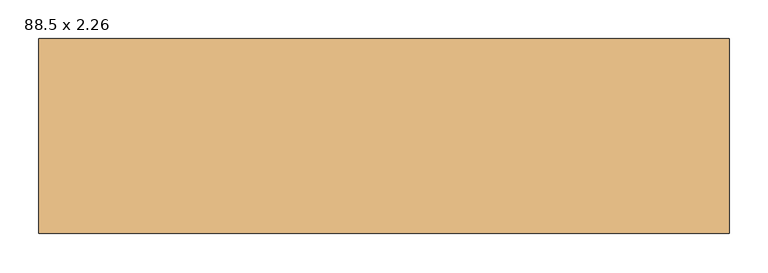
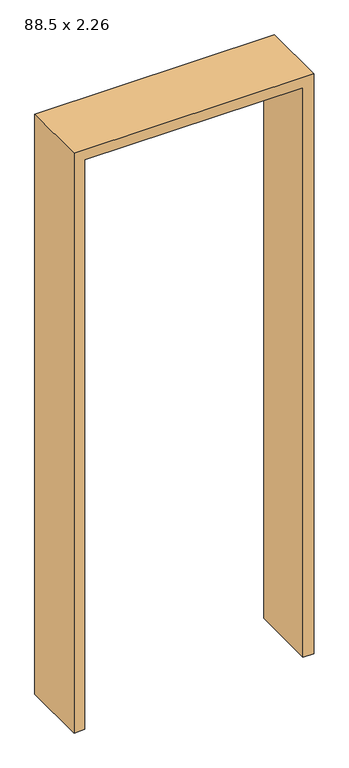
"""IFC4 building model written with IfcOpenShell, lengths in millimetres: door geometry, Durchfahrt - Blockzarge : 88.5 x 2.26."""

import ifcopenshell
import ifcopenshell.guid

model = None  # the IFC model being written
_history = None  # IfcOwnerHistory: only IFC2X3 demands one
_inside = {}  # id of a spatial element -> (the spatial element, [elements in it])
_under = {}  # id of a project, library or spatial element -> (it, [spatial elements below it])
_declared = {}  # id of a project -> (the project, [libraries it declares])
_typed = {}  # id of a type object -> (the type object, [elements of that type])
_made_of = {}  # id of a material, layer set ... -> (it, [elements and type objects made of it])


def new_model(schema):
    """Start an empty IFC model of exactly this schema.

    Asked for "IFC4X3", IfcOpenShell would pick the latest addendum, in which some entities
    have other attributes; the version numbers below select the first issue.
    IFC2X3 requires an IfcOwnerHistory on every rooted entity: one is made here for all.
    """
    global model, _history
    if schema == "IFC4X3":
        model = ifcopenshell.file(schema_version=(4, 3, 0, 0))
    else:
        model = ifcopenshell.file(schema=schema)
    _inside.clear()
    _under.clear()
    _declared.clear()
    _typed.clear()
    _made_of.clear()
    _history = None
    if model.schema == "IFC2X3":
        org = make("IfcOrganization", Name="unknown")
        user = make(
            "IfcPersonAndOrganization",
            ThePerson=make("IfcPerson", FamilyName="unknown"),
            TheOrganization=org,
        )
        app = make(
            "IfcApplication",
            ApplicationDeveloper=org,
            Version="unknown",
            ApplicationFullName="unknown",
            ApplicationIdentifier="unknown",
        )
        _history = make(
            "IfcOwnerHistory",
            OwningUser=user,
            OwningApplication=app,
            ChangeAction="ADDED",
            CreationDate=0,
        )
    return model


def make(cls, **values):
    """One entity of the class cls with the attributes given. An attribute that is None is left unset."""
    return model.create_entity(
        cls, **{name: value for name, value in values.items() if value is not None}
    )


def rooted(cls, **values):
    """An entity with a GlobalId (a new one), such as an element, a storey or a relation."""
    return make(cls, GlobalId=ifcopenshell.guid.new(), OwnerHistory=_history, **values)


def si_unit(unit_type, name, prefix=None):
    """IfcSIUnit, for example si_unit("LENGTHUNIT", "METRE", prefix="MILLI")."""
    return make("IfcSIUnit", UnitType=unit_type, Prefix=prefix, Name=name)


def assignment(units):
    """IfcUnitAssignment: the units of a project."""
    return None if units is None else make("IfcUnitAssignment", Units=units)


def point(xyz):
    """IfcCartesianPoint."""
    return None if xyz is None else make("IfcCartesianPoint", Coordinates=xyz)


def direction(xyz):
    """IfcDirection."""
    return None if xyz is None else make("IfcDirection", DirectionRatios=xyz)


def frame(location, z_axis=None, x_axis=None):
    """IfcAxis2Placement3D, a coordinate frame: its origin and axes. An axis left out is left unset."""
    return make(
        "IfcAxis2Placement3D",
        Location=point(location),
        Axis=direction(z_axis),
        RefDirection=direction(x_axis),
    )


def origin():
    """The frame at (0, 0, 0) with its axes left unset."""
    return frame((0.0, 0.0, 0.0))


def place(relative_to, where):
    """IfcLocalPlacement: puts the frame where relative to a parent placement (None: the world)."""
    return make(
        "IfcLocalPlacement", PlacementRelTo=relative_to, RelativePlacement=where
    )


def context(
    kind, dimensions, precision=None, world=None, true_north=None, identifier=None
):
    """IfcGeometricRepresentationContext, for example the 3D "Model" context."""
    return make(
        "IfcGeometricRepresentationContext",
        ContextIdentifier=identifier,
        ContextType=kind,
        CoordinateSpaceDimension=dimensions,
        Precision=precision,
        WorldCoordinateSystem=world,
        TrueNorth=true_north,
    )


def project(units=None, contexts=None):
    """IfcProject with its units and contexts."""
    return rooted(
        "IfcProject",
        Name="project",
        RepresentationContexts=contexts,
        UnitsInContext=assignment(units),
    )


def spatial(cls, under=None, at=None, **own):
    """A site, building, storey or space (cls), placed at a placement, below another one or the project."""
    s = rooted(cls, ObjectPlacement=at, **own)
    if under is not None:
        _under.setdefault(under.id(), (under, []))[1].append(s)
    return s


def polyline(points):
    """IfcPolyline through the points."""
    return make("IfcPolyline", Points=[point(p) for p in points])


def outline(outer, holes=None, kind="AREA"):
    """IfcArbitraryClosedProfileDef: a profile drawn as a closed curve; with holes, ...WithVoids."""
    if holes is None:
        return make("IfcArbitraryClosedProfileDef", ProfileType=kind, OuterCurve=outer)
    return make(
        "IfcArbitraryProfileDefWithVoids",
        ProfileType=kind,
        OuterCurve=outer,
        InnerCurves=holes,
    )


def extrude(swept, where, along, depth):
    """IfcExtrudedAreaSolid: the profile swept, set in the frame where, extruded along a direction by depth."""
    return make(
        "IfcExtrudedAreaSolid",
        SweptArea=swept,
        Position=where,
        ExtrudedDirection=direction(along),
        Depth=depth,
    )


def shape(context_of_items, identifier, shape_type, items):
    """IfcShapeRepresentation: the items that make up one representation, for example the "Body"."""
    return make(
        "IfcShapeRepresentation",
        ContextOfItems=context_of_items,
        RepresentationIdentifier=identifier,
        RepresentationType=shape_type,
        Items=items,
    )


def source(mapping_origin, context_of_items, identifier, shape_type, items):
    """IfcRepresentationMap: a shape defined once, which mapped items show again and again."""
    return make(
        "IfcRepresentationMap",
        MappingOrigin=mapping_origin,
        MappedRepresentation=shape(context_of_items, identifier, shape_type, items),
    )


def transform(
    local_origin,
    x_axis=None,
    y_axis=None,
    z_axis=None,
    scale=None,
    scale2=None,
    scale3=None,
    uniform=True,
):
    """IfcCartesianTransformationOperator3D, or its non-uniform kind. x_axis, y_axis, z_axis: its Axis1, 2, 3."""
    if uniform:
        return make(
            "IfcCartesianTransformationOperator3D",
            Axis1=direction(x_axis),
            Axis2=direction(y_axis),
            LocalOrigin=point(local_origin),
            Scale=scale,
            Axis3=direction(z_axis),
        )
    return make(
        "IfcCartesianTransformationOperator3DnonUniform",
        Axis1=direction(x_axis),
        Axis2=direction(y_axis),
        LocalOrigin=point(local_origin),
        Scale=scale,
        Axis3=direction(z_axis),
        Scale2=scale2,
        Scale3=scale3,
    )


def mapped(mapping_source, mapping_target):
    """IfcMappedItem: shows the shape of a source again, moved by a transform."""
    return make(
        "IfcMappedItem", MappingSource=mapping_source, MappingTarget=mapping_target
    )


def made_of(thing, what):
    """Note that an element or type object is made of a material, layer set ...; save() writes the relation."""
    if what is not None:
        _made_of.setdefault(what.id(), (what, []))[1].append(thing)
    return thing


def element(
    cls,
    number,
    at=None,
    inside=None,
    cuts=None,
    type_object=None,
    material=None,
    context=None,
    identifier="Body",
    shape_type=None,
    held_by="IfcProductDefinitionShape",
    body=None,
    shapes=None,
    **own,
):
    """One element of the class cls, such as IfcWall. Its Tag is "e" and its number.

    at: its placement. inside: the storey or other place that contains it. cuts: it is an
    opening in that element (IfcRelVoidsElement). A single representation is given by context,
    identifier, shape_type and body (its items); several are given by shapes. held_by: the class
    of the entity that holds the representations. save() writes the other relations.
    """
    e = rooted(cls, Tag="e%d" % number, ObjectPlacement=at, **own)
    if body is not None:
        shapes = [shape(context, identifier, shape_type, body)]
    if shapes is not None:
        e.Representation = make(held_by, Representations=shapes)
    if inside is not None:
        _inside.setdefault(inside.id(), (inside, []))[1].append(e)
    if cuts is not None:
        rooted(
            "IfcRelVoidsElement", RelatingBuildingElement=cuts, RelatedOpeningElement=e
        )
    if type_object is not None:
        _typed.setdefault(type_object.id(), (type_object, []))[1].append(e)
    return made_of(e, material)


def aggregate(whole, parts):
    """IfcRelAggregates: a whole, such as a stair, and the parts it consists of."""
    return rooted("IfcRelAggregates", RelatingObject=whole, RelatedObjects=parts)


def save(model, path):
    """Write the relations noted so far, then the file.

    IfcRelAggregates (storeys below a building ...), IfcRelContainedInSpatialStructure (elements
    in a storey), IfcRelDefinesByType, IfcRelAssociatesMaterial and IfcRelDeclares: one each for
    every whole, place, type object, material and project.
    """
    for whole, parts in _under.values():
        aggregate(whole, parts)
    for where, things in _inside.values():
        rooted(
            "IfcRelContainedInSpatialStructure",
            RelatedElements=things,
            RelatingStructure=where,
        )
    for kind, things in _typed.values():
        rooted("IfcRelDefinesByType", RelatedObjects=things, RelatingType=kind)
    for what, things in _made_of.values():
        rooted("IfcRelAssociatesMaterial", RelatedObjects=things, RelatingMaterial=what)
    for by, libraries in _declared.values():
        rooted("IfcRelDeclares", RelatingContext=by, RelatedDefinitions=libraries)
    model.write(path)


def door_88_5_x_2_26_cc2fa13a(model_context):
    return source(origin(), model_context, "Body", "SweptSolid", [
        extrude(outline(polyline([(2360.0, 442.5), (2360.0, -442.5), (100.0, -442.5), (100.0, -402.5), (2320.0, -402.5), (2320.0, 402.5), (100.0, 402.5), (100.0, 442.5), (2360.0, 442.5)])), frame((0.0, -110.5653859, 0.0), z_axis=(0.0, 1.0, 0.0), x_axis=(0.0, 0.0, 1.0)), (0.0, 0.0, 1.0), 250.0),
    ])


if __name__ == "__main__":
    model = new_model("IFC4")
    model_context = context("Model", 3, world=origin())
    ifc_project = project(units=[si_unit("LENGTHUNIT", "METRE", prefix="MILLI")], contexts=[model_context])
    site = spatial("IfcSite", under=ifc_project)
    building = spatial("IfcBuilding", under=site)
    placement = place(None, origin())
    door_88_5_x_2_26_shape = door_88_5_x_2_26_cc2fa13a(model_context)
    element("IfcDoor", 1, ObjectType="Durchfahrt - Blockzarge : 88.5 x 2.26", at=placement, inside=building, context=model_context, shape_type="MappedRepresentation", body=[
        mapped(door_88_5_x_2_26_shape, transform((0.0, 0.0, 0.0), x_axis=(1.0, 0.0, 0.0), y_axis=(0.0, 1.0, 0.0), z_axis=(0.0, 0.0, 1.0))),
    ])
    save(model, "model.ifc")

# Revit data of these elements
# Type "Durchfahrt - Blockzarge : 88.5 x 2.26"
#   Type Mark = "23"
#   Keynote = "16.03"
#   Rough Width = 0.885 m
#   Stärke Futter = 0.040 m
#   Rough Height [instance default] = 2.360 m
#   Height = 2.260 m
#   Fußbodenaufbau [instance default] = 0.100 m
#   Width = 0.885 m
#   Sichtbarkeit Sturzlinien [instance default] = yes
#   Rahmen/Pfosten = none
#   Function = (empty or 0)
#   Wall Closure = (empty or 0)
# Element 1 (IfcDoor, "Durchfahrt - Blockzarge : 88.5 x 2.26")
#   Materials on its faces: "Holz - Birke"
# Materials
#   "Holz - Birke": class "Holz", colour RGB 213 164 103, transparency 0, Cost = 0
